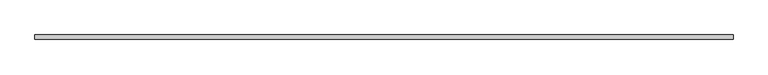
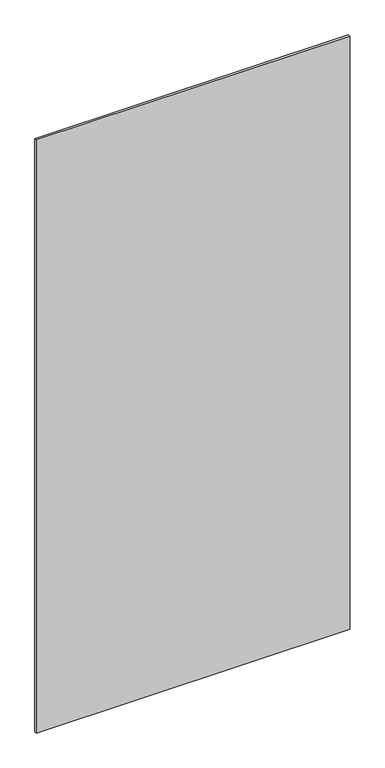
"""IFC4 building model written with IfcOpenShell, lengths in millimetres: proxy geometry, Panel:Panel:300402:Panel:300402 : Panel:Panel:300402:300124:Panel:300402:Panel:300402 : Panel:Panel:300402:300124 : Panel:Panel:300402:Panel:300402 : Panel:Panel:300402:300124:5 : Panel:Panel:300402:Panel:300402 : Panel:Panel:300402:300124:Panel:300402:Panel:300402 : Panel:Panel:300402:300124 : Panel:Panel:300402:Panel:300402 : Panel:Panel:300402:300124:300083."""

from ifc_helpers import new_model, si_unit, frame, origin, place, context, project, spatial, polyline, outline, extrude, source, transform, mapped, element, save


def generic_models_62b7404d(model_context):
    return source(origin(), model_context, "Body", "SweptSolid", [
        extrude(outline(polyline([(570452.6367239, -579076.8913841), (571671.8367239, -579076.8913841), (571671.8367239, -579084.8288841), (570452.6367239, -579084.8288841), (570452.6367239, -579076.8913841)])), frame((0.0, 0.0, 25.4), z_axis=(0.0, 0.0, 1.0), x_axis=(1.0, 0.0, 0.0)), (0.0, 0.0, 1.0), 2438.4),
    ])


if __name__ == "__main__":
    model = new_model("IFC4")
    model_context = context("Model", 3, world=origin())
    ifc_project = project(units=[si_unit("LENGTHUNIT", "METRE", prefix="MILLI")], contexts=[model_context])
    site = spatial("IfcSite", under=ifc_project)
    building = spatial("IfcBuilding", under=site)
    placement = place(None, origin())
    generic_models_shape = generic_models_62b7404d(model_context)
    element("IfcBuildingElementProxy", 1, Name="Panel:Panel:300402:Panel:300402 : Panel:Panel:300402:300124:Panel:300402:Panel:300402 : Panel:Panel:300402:300124 : Panel:Panel:300402:Panel:300402 : Panel:Panel:300402:300124:5 : Panel:Panel:300402:Panel:300402 : Panel:Panel:300402:300124:Panel:300402:Panel:300402 : Panel:Panel:300402:300124 : Panel:Panel:300402:Panel:300402 : Panel:Panel:300402:300124:300083", ObjectType="Panel:Panel:300402:Panel:300402 : Panel:Panel:300402:300124:Panel:300402:Panel:300402 : Panel:Panel:300402:300124 : Panel:Panel:300402:Panel:300402 : Panel:Panel:300402:300124:5 : Panel:Panel:300402:Panel:300402 : Panel:Panel:300402:300124:Panel:300402:Panel:300402 : Panel:Panel:300402:300124 : Panel:Panel:300402:Panel:300402 : Panel:Panel:300402:300124:300083", at=placement, inside=building, context=model_context, shape_type="MappedRepresentation", body=[
        mapped(generic_models_shape, transform((0.0, 0.0, 0.0), x_axis=(1.0, 0.0, 0.0), y_axis=(0.0, 1.0, 0.0), z_axis=(0.0, 0.0, 1.0))),
    ])
    save(model, "model.ifc")

# Revit data of these elements
# Type "Panel:Panel:300402:Panel:300402 : Panel:Panel:300402:300124:Panel:300402:Panel:300402 : Panel:Panel:300402:300124 : Panel:Panel:300402:Panel:300402 : Panel:Panel:300402:300124:5 : Panel:Panel:300402:Panel:300402 : Panel:Panel:300402:300124:Panel:300402:Panel:300402 : Panel:Panel:300402:300124 : Panel:Panel:300402:Panel:300402 : Panel:Panel:300402:300124:300083"
#   NameOverride = "Panel:Panel:300402:Panel:300402 : Panel:Panel:300402:300124:Panel:300402:Panel:300402 : Panel:Panel:300402:300124 : Panel:Panel:300402:Panel:300402 : Panel:Panel:300402:300124:300083"
#   ObjectTypeOverride = "Panel:300402:Panel:300402 : Panel:Panel:300402:300124 : Panel:Panel:300402:Panel:300402 : Panel:Panel:300402:300124"
#   Reference = "Panel"
#   Tag = "300083"
# Element 1 (IfcBuildingElementProxy, "Panel:Panel:300402:Panel:300402 : Panel:Panel:300402:300124:Panel:300402:Panel:300402 : Panel:Panel:300402:300124 : Panel:Panel:300402:Panel:300402 : Panel:Panel:300402:300124:5 : Panel:Panel:300402:Panel:300402 : Panel:Panel:300402:300124:Panel:300402:Panel:300402 : Panel:Panel:300402:300124 : Panel:Panel:300402:Panel:300402 : Panel:Panel:300402:300124:300083")
#   Materials on its faces: "5/16\" PHENOLIC RESIN PANELS (CLASS A FLAME SPREAD) - EXPOSED FASTENERS"
# Materials
#   "5/16\" PHENOLIC RESIN PANELS (CLASS A FLAME SPREAD) - EXPOSED FASTENERS": class "Unassigned", colour RGB 64 64 64, transparency 0, Keynote = "M07420000.01", Cost = 0
